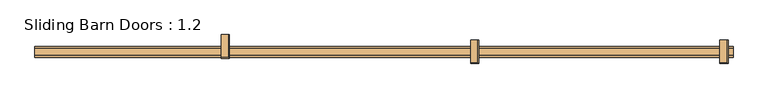
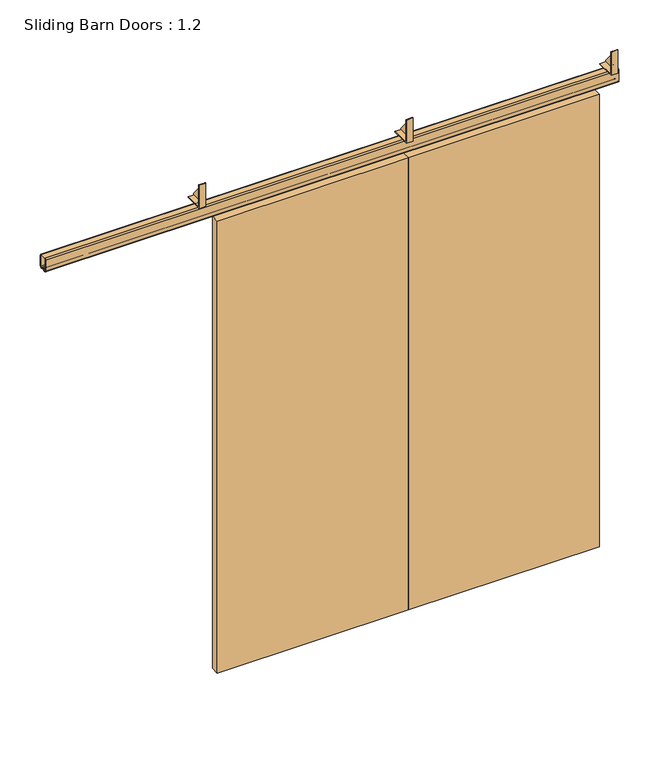
"""IFC4 building model written with IfcOpenShell, lengths in millimetres: door geometry, Sliding Barn Doors : 1.2."""

from ifc_helpers import new_model, si_unit, point, frame, frame_2d, origin, place, context, project, spatial, polyline, circle_curve, trimmed, segment, composite_curve, outline, extrude, source, transform, mapped, element, save


def sliding_barn_doors_1_2_d088c784(model_context):
    return source(origin(), model_context, "Body", "SweptSolid", [
        extrude(outline(polyline([(158.75, 2152.65), (158.75, 2146.3), (79.375, 2146.3), (79.375, 2247.773), (158.75, 2152.65)])), frame((-1354.9808594, 0.0, 0.0), z_axis=(1.0, 0.0, 0.0), x_axis=(0.0, 1.0, 0.0)), (0.0, 0.0, 1.0), 3.175),
        extrude(outline(polyline([(76.2, 2143.125), (76.2, 2247.773), (79.375, 2247.773), (79.375, 2146.3), (158.75, 2146.3), (158.75, 2143.125), (76.2, 2143.125)])), frame((-1380.2816406, 0.0, 0.0), z_axis=(1.0, 0.0, 0.0), x_axis=(0.0, 1.0, 0.0)), (0.0, 0.0, 1.0), 28.4757812),
        extrude(outline(polyline([(139.7, 2152.65), (139.7, 2146.3), (60.325, 2146.3), (60.325, 2247.773), (139.7, 2152.65)])), frame((-484.2371094, 0.0, 0.0), z_axis=(1.0, 0.0, 0.0), x_axis=(0.0, 1.0, 0.0)), (0.0, 0.0, 1.0), 3.175),
        extrude(outline(polyline([(57.15, 2143.125), (57.15, 2247.773), (60.325, 2247.773), (60.325, 2146.3), (139.7, 2146.3), (139.7, 2143.125), (57.15, 2143.125)])), frame((-509.5378906, 0.0, 0.0), z_axis=(1.0, 0.0, 0.0), x_axis=(0.0, 1.0, 0.0)), (0.0, 0.0, 1.0), 28.4757813),
        extrude(outline(polyline([(139.7, 2152.65), (139.7, 2146.3), (60.325, 2146.3), (60.325, 2247.773), (139.7, 2152.65)])), frame((386.5066406, 0.0, 0.0), z_axis=(1.0, 0.0, 0.0), x_axis=(0.0, 1.0, 0.0)), (0.0, 0.0, 1.0), 3.175),
        extrude(outline(polyline([(57.15, 2143.125), (57.15, 2247.773), (60.325, 2247.773), (60.325, 2146.3), (139.7, 2146.3), (139.7, 2143.125), (57.15, 2143.125)])), frame((361.2058594, 0.0, 0.0), z_axis=(1.0, 0.0, 0.0), x_axis=(0.0, 1.0, 0.0)), (0.0, 0.0, 1.0), 28.4757813),
        extrude(outline(polyline([(-1199.61025, 117.475), (-1148.30225, 117.475), (-1148.30225, 114.3), (-1199.61025, 114.3), (-1199.61025, 117.475)])), frame((0.0, 0.0, 1889.252), z_axis=(0.0, 0.0, 1.0), x_axis=(1.0, 0.0, 0.0)), (0.0, 0.0, 1.0), 168.148),
        extrude(outline(polyline([(-640.81025, 117.475), (-589.50225, 117.475), (-589.50225, 114.3), (-640.81025, 114.3), (-640.81025, 117.475)])), frame((0.0, 0.0, 1889.252), z_axis=(0.0, 0.0, 1.0), x_axis=(1.0, 0.0, 0.0)), (0.0, 0.0, 1.0), 168.148),
        extrude(outline(polyline([(-386.81025, 117.475), (-335.50225, 117.475), (-335.50225, 114.3), (-386.81025, 114.3), (-386.81025, 117.475)])), frame((0.0, 0.0, 1889.252), z_axis=(0.0, 0.0, 1.0), x_axis=(1.0, 0.0, 0.0)), (0.0, 0.0, 1.0), 168.148),
        extrude(outline(polyline([(171.98975, 117.475), (223.29775, 117.475), (223.29775, 114.3), (171.98975, 114.3), (171.98975, 117.475)])), frame((0.0, 0.0, 1889.252), z_axis=(0.0, 0.0, 1.0), x_axis=(1.0, 0.0, 0.0)), (0.0, 0.0, 1.0), 168.148),
        extrude(outline(polyline([(-1300.95625, 114.3), (-488.15625, 114.3), (-488.15625, 79.375), (-1300.95625, 79.375), (-1300.95625, 114.3)])), frame((0.0, 0.0, 25.4), z_axis=(0.0, 0.0, 1.0), x_axis=(1.0, 0.0, 0.0)), (0.0, 0.0, 1.0), 2032.0),
        extrude(outline(polyline([(-488.15625, 114.3), (324.64375, 114.3), (324.64375, 79.375), (-488.15625, 79.375), (-488.15625, 114.3)])), frame((0.0, 0.0, 25.4), z_axis=(0.0, 0.0, 1.0), x_axis=(1.0, 0.0, 0.0)), (0.0, 0.0, 1.0), 2032.0),
        extrude(outline(composite_curve([segment(polyline([(85.725, 2143.125), (111.252, 2143.125)]), True, "CONTINUOUS"), segment(trimmed(circle_curve(frame_2d((111.252, 2136.775)), 6.35), [point((111.252, 2143.125))], [point((117.602, 2136.775))], False, "CARTESIAN"), True, "CONTINUOUS"), segment(polyline([(117.602, 2136.775), (117.602, 2088.515)]), True, "CONTINUOUS"), segment(trimmed(circle_curve(frame_2d((111.252, 2088.515)), 6.35), [point((117.602, 2088.515))], [point((111.252, 2082.165))], False, "CARTESIAN"), True, "CONTINUOUS"), segment(polyline([(111.252, 2082.165), (105.8433147, 2082.165)]), True, "CONTINUOUS"), segment(trimmed(circle_curve(frame_2d((105.8433147, 2083.7525)), 1.5875), [point((105.8433147, 2082.165))], [point((104.2849816, 2083.4495907))], False, "CARTESIAN"), True, "CONTINUOUS"), segment(polyline([(104.2849816, 2083.4495907), (102.8594659, 2090.7832331), (104.3756029, 2090.7832331), (105.7615251, 2083.6532812), (111.252, 2083.6532812)]), True, "CONTINUOUS"), segment(trimmed(circle_curve(frame_2d((111.252, 2088.515)), 4.8617187), [point((111.252, 2083.6532812))], [point((116.1137188, 2088.515))], True, "CARTESIAN"), True, "CONTINUOUS"), segment(polyline([(116.1137188, 2088.515), (116.1137188, 2136.775)]), True, "CONTINUOUS"), segment(trimmed(circle_curve(frame_2d((111.252, 2136.775)), 4.8617187), [point((116.1137188, 2136.775))], [point((111.252, 2141.6367187))], True, "CARTESIAN"), True, "CONTINUOUS"), segment(polyline([(111.252, 2141.6367187), (85.725, 2141.6367187)]), True, "CONTINUOUS"), segment(trimmed(circle_curve(frame_2d((85.725, 2136.775)), 4.8617187), [point((85.725, 2141.6367187))], [point((80.8632813, 2136.775))], True, "CARTESIAN"), True, "CONTINUOUS"), segment(polyline([(80.8632813, 2136.775), (80.8632813, 2088.515)]), True, "CONTINUOUS"), segment(trimmed(circle_curve(frame_2d((85.725, 2088.515)), 4.8617187), [point((80.8632813, 2088.515))], [point((85.725, 2083.6532812))], True, "CARTESIAN"), True, "CONTINUOUS"), segment(polyline([(85.725, 2083.6532812), (91.2154749, 2083.6532812), (92.6013971, 2090.7832331), (94.1175341, 2090.7832331), (92.6920184, 2083.4495907)]), True, "CONTINUOUS"), segment(trimmed(circle_curve(frame_2d((91.1336853, 2083.7525)), 1.5875), [point((92.6920184, 2083.4495907))], [point((91.1336853, 2082.165))], False, "CARTESIAN"), True, "CONTINUOUS"), segment(polyline([(91.1336853, 2082.165), (85.725, 2082.165)]), True, "CONTINUOUS"), segment(trimmed(circle_curve(frame_2d((85.725, 2088.515)), 6.35), [point((85.725, 2082.165))], [point((79.375, 2088.515))], False, "CARTESIAN"), True, "CONTINUOUS"), segment(polyline([(79.375, 2088.515), (79.375, 2136.775)]), True, "CONTINUOUS"), segment(trimmed(circle_curve(frame_2d((85.725, 2136.775)), 6.35), [point((79.375, 2136.775))], [point((85.725, 2143.125))], False, "CARTESIAN"), True, "CONTINUOUS")], self_intersect=False)), frame((-2031.20625, 0.0, 0.0), z_axis=(1.0, 0.0, 0.0), x_axis=(0.0, 1.0, 0.0)), (0.0, 0.0, 1.0), 2438.4),
    ])


if __name__ == "__main__":
    model = new_model("IFC4")
    model_context = context("Model", 3, world=origin())
    ifc_project = project(units=[si_unit("LENGTHUNIT", "METRE", prefix="MILLI")], contexts=[model_context])
    site = spatial("IfcSite", under=ifc_project)
    building = spatial("IfcBuilding", under=site)
    placement = place(None, origin())
    sliding_barn_doors_1_2_shape = sliding_barn_doors_1_2_d088c784(model_context)
    element("IfcDoor", 1, ObjectType="Sliding Barn Doors : 1.2", at=placement, inside=building, context=model_context, shape_type="MappedRepresentation", body=[
        mapped(sliding_barn_doors_1_2_shape, transform((0.0, 0.0, 0.0), x_axis=(1.0, 0.0, 0.0), y_axis=(0.0, 1.0, 0.0), z_axis=(0.0, 0.0, 1.0))),
    ])
    save(model, "model.ifc")

# Revit data of these elements
# Type "Sliding Barn Doors : 1.2"
#   Type Mark = "44"
#   Analytic Construction = "<None>"
#   rail_overlap_left = 0' - 5 1/4"
#   rail_length = 8' - 0"
#   overlap_left = 0' - 2"
#   overlap = 0' - 0"
#   bracket_right = 3' - 7"
#   bracket_left = 0' - 4"
#   Thickness = 0' - 1 3/8"
#   Panel Width = 2' - 8"
#   Panel Height = 6' - 8"
#   Gap 2 = 0' - 0 1/2"
#   Gap 1 = 0' - 0 7/8"
#   Frame Projection Ext. = 0' - 1"
#   Frame Projection Int. = 0' - 1"
#   Frame Width = 0' - 3"
#   Height = 6' - 4"
#   Width = 1' - 9 9/16"
#   Bracket_offset = 0' - 5"
#   Door_4 = no
#   Door_3 = no
#   Hardware Material = Metal - Aluminum
#   Door Material = Closet_1
#   Function = (empty or 0)
#   Wall Closure = (empty or 0)
# Element 1 (IfcDoor, "Sliding Barn Doors : 1.2")
#   Materials on its faces: "Metal - Aluminum", "Closet_1"
# Materials
#   "Metal - Aluminum": class "Metal", colour RGB 247 247 247, transparency 0
#   "Closet_1": class "Paint", colour RGB 58 62 47, transparency 0, Cost = 0
